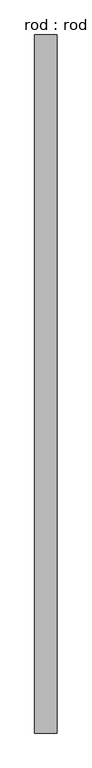
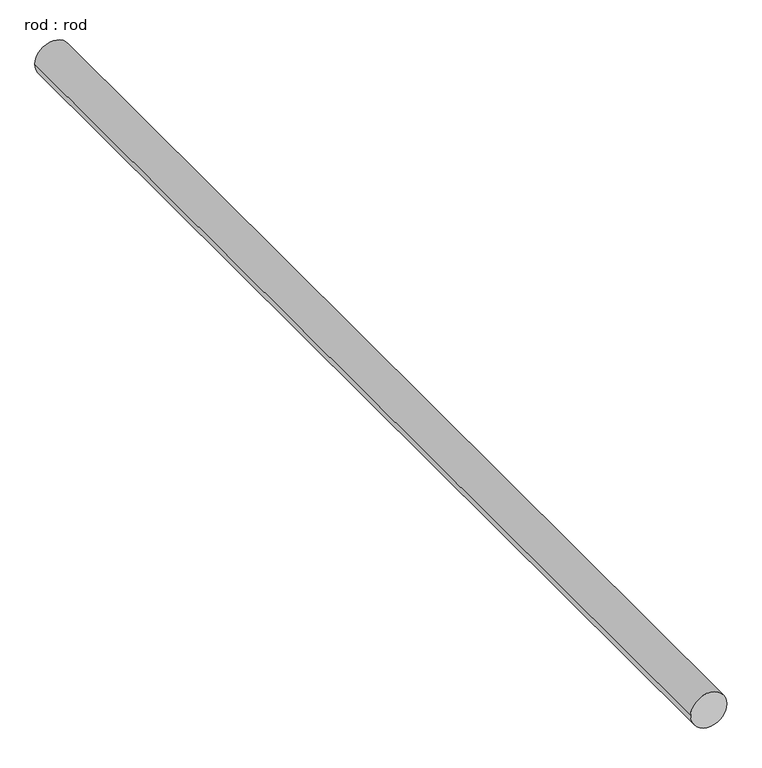
"""IFC4 building model written with IfcOpenShell, lengths in millimetres: proxy geometry, rod : rod."""

from ifc_helpers import new_model, si_unit, point, frame, frame_2d, origin, place, context, project, spatial, circle_curve, trimmed, segment, composite_curve, outline, extrude, source, transform, mapped, element, save


def rod_rod_71858249(model_context):
    return source(origin(), model_context, "Body", "SweptSolid", [
        extrude(outline(composite_curve([segment(trimmed(circle_curve(frame_2d((0.0108462, 0.0)), 200.0), [point((0.0108462, 200.0))], [point((0.0108462, -200.0))], False, "CARTESIAN"), True, "CONTINUOUS"), segment(trimmed(circle_curve(frame_2d((0.0108462, 0.0)), 200.0), [point((0.0108462, -200.0))], [point((0.0108462, 200.0))], False, "CARTESIAN"), True, "CONTINUOUS")], self_intersect=False)), frame((0.0, -2172.9816499, 0.0), z_axis=(0.0, 1.0, 0.0), x_axis=(0.0, 0.0, 1.0)), (0.0, 0.0, 1.0), 12531.4205304),
    ])


if __name__ == "__main__":
    model = new_model("IFC4")
    model_context = context("Model", 3, world=origin())
    ifc_project = project(units=[si_unit("LENGTHUNIT", "METRE", prefix="MILLI")], contexts=[model_context])
    site = spatial("IfcSite", under=ifc_project)
    building = spatial("IfcBuilding", under=site)
    placement = place(None, origin())
    rod_rod_shape = rod_rod_71858249(model_context)
    element("IfcBuildingElementProxy", 1, Name="rod : rod", ObjectType="rod : rod", at=placement, inside=building, context=model_context, shape_type="MappedRepresentation", body=[
        mapped(rod_rod_shape, transform((0.0, 0.0, 0.0), x_axis=(1.0, 0.0, 0.0), y_axis=(0.0, 1.0, 0.0), z_axis=(0.0, 0.0, 1.0))),
    ])
    save(model, "model.ifc")

# Revit data of these elements
# Type "rod : rod"
#   Default Elevation = 0
